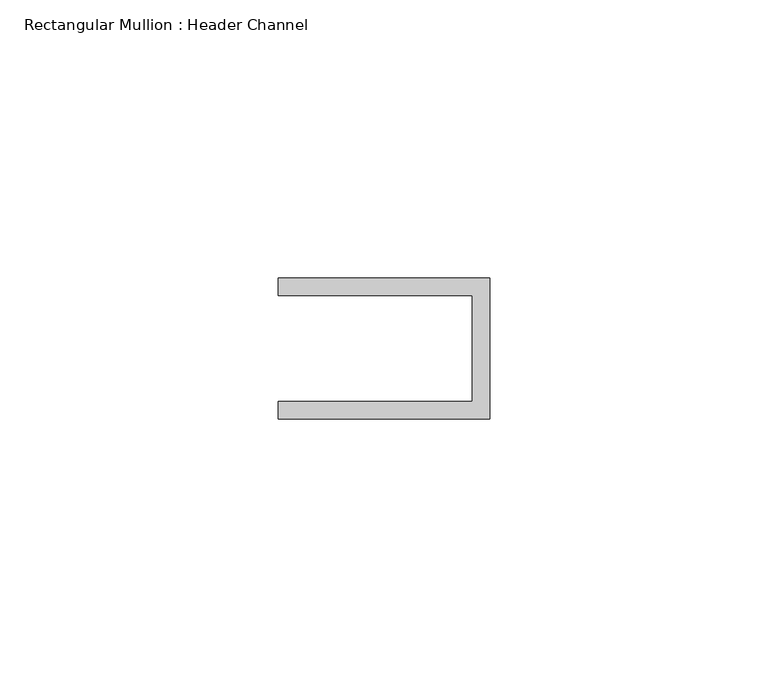
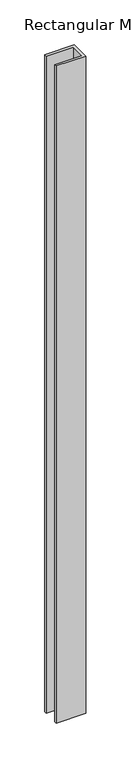
"""IFC4 building model written with IfcOpenShell, lengths in millimetres: member geometry, Rectangular Mullion : Header Channel."""

from ifc_helpers import new_model, si_unit, frame, origin, place, context, project, spatial, polyline, outline, extrude, source, transform, mapped, element, save


def rectangular_mullion_header_channel_a241ad57(model_context):
    return source(origin(), model_context, "Body", "SweptSolid", [
        extrude(outline(polyline([(0.0, -12.7), (-38.1, -12.7), (-38.1, -9.525), (-3.175, -9.525), (-3.175, 9.525), (-38.1, 9.525), (-38.1, 12.7), (0.0, 12.7), (0.0, -12.7)])), frame((0.0, 0.0, -894.320152), z_axis=(0.0, 0.0, 1.0), x_axis=(1.0, 0.0, 0.0)), (0.0, 0.0, 1.0), 894.320152),
    ])


if __name__ == "__main__":
    model = new_model("IFC4")
    model_context = context("Model", 3, world=origin())
    ifc_project = project(units=[si_unit("LENGTHUNIT", "METRE", prefix="MILLI")], contexts=[model_context])
    site = spatial("IfcSite", under=ifc_project)
    building = spatial("IfcBuilding", under=site)
    placement = place(None, origin())
    rectangular_mullion_header_channel_shape = rectangular_mullion_header_channel_a241ad57(model_context)
    element("IfcMember", 1, ObjectType="Rectangular Mullion : Header Channel", at=placement, inside=building, context=model_context, shape_type="MappedRepresentation", body=[
        mapped(rectangular_mullion_header_channel_shape, transform((0.0, 0.0, 0.0), x_axis=(1.0, 0.0, 0.0), y_axis=(0.0, 1.0, 0.0), z_axis=(0.0, 0.0, 1.0))),
    ])
    save(model, "model.ifc")

# Revit data of these elements
# Type "Rectangular Mullion : Header Channel"
#   built-in parameter 1007322 = 0.0833333 (stored number, unit not read)
#   built-in parameter 1007321 = -0.03125 (stored number, unit not read)
#   built-in parameter 1007320 = 0.0416667 (stored number, unit not read)
# Element 1 (IfcMember, "Rectangular Mullion : Header Channel")
#   Materials on its faces: "ALUM"
# Materials
#   "ALUM": class "Generic", colour RGB 157 157 157, transparency 0, Cost = 0
